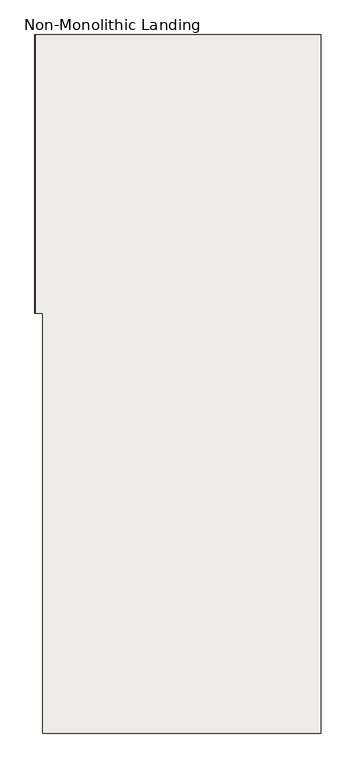
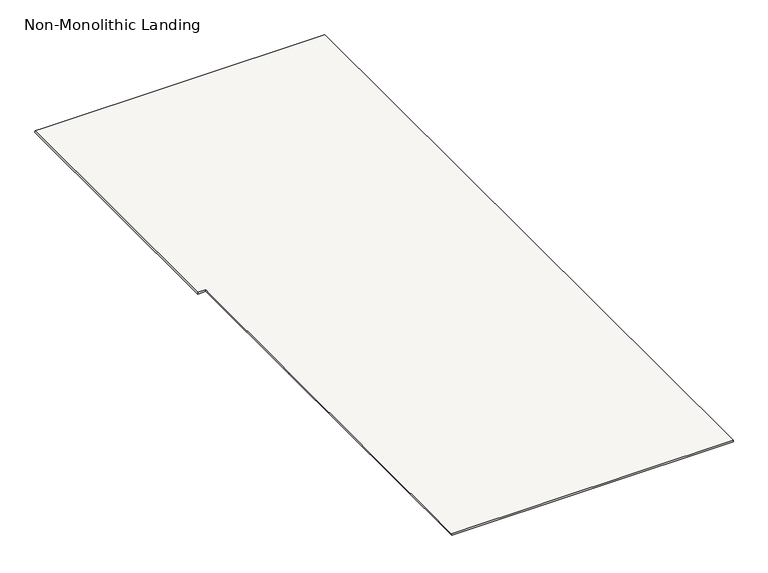
"""IFC4 building model written with IfcOpenShell, lengths in millimetres: slab geometry, Non-Monolithic Landing."""

from ifc_helpers import new_model, si_unit, origin, place, context, project, spatial, faceted_brep, source, transform, mapped, element, save


def non_monolithic_landing_193fae1a(model_context):
    return source(origin(), model_context, "Body", "Brep", [
        faceted_brep([(16318.9400908, 13130.4345331, 9941.1764706), (16318.0900908, 13130.4345331, 9935.1764706), (16318.0900908, 12030.4345331, 9935.1764706), (16318.9400908, 12030.4345331, 9941.1764706), (16350.0, 10370.4345331, 9941.1764706), (17450.0, 10370.4345331, 9941.1764706), (17450.0, 13130.4345331, 9941.1764706), (16350.0, 13130.4345331, 9941.1764706), (16350.0, 12030.4345331, 9941.1764706), (16350.0, 11470.4345331, 9941.1764706), (17450.0, 13130.4345331, 9935.1764706), (17450.0, 10370.4345331, 9935.1764706), (16350.85, 10370.4345331, 9935.1764706), (16350.85, 11470.4345331, 9935.1764706), (16350.0, 11470.4345331, 9935.1764706), (16350.0, 12030.4345331, 9935.1764706), (16350.0, 13130.4345331, 9935.1764706)], [[[0, 1, 2, 3]], [[4, 5, 6, 7, 0, 3, 8, 9]], [[10, 11, 12, 13, 14, 15, 2, 1, 16]], [[9, 8, 15, 14]], [[0, 7, 16, 1]], [[7, 6, 10, 16]], [[6, 5, 11, 10]], [[5, 4, 12, 11]], [[13, 9, 14]], [[9, 13, 12, 4]], [[8, 3, 2, 15]]]),
    ])


if __name__ == "__main__":
    model = new_model("IFC4")
    model_context = context("Model", 3, world=origin())
    ifc_project = project(units=[si_unit("LENGTHUNIT", "METRE", prefix="MILLI")], contexts=[model_context])
    site = spatial("IfcSite", under=ifc_project)
    building = spatial("IfcBuilding", under=site)
    placement = place(None, origin())
    non_monolithic_landing_shape = non_monolithic_landing_193fae1a(model_context)
    element("IfcSlab", 1, ObjectType="Non-Monolithic Landing", at=placement, inside=building, context=model_context, shape_type="MappedRepresentation", body=[
        mapped(non_monolithic_landing_shape, transform((0.0, 0.0, 0.0), x_axis=(1.0, 0.0, 0.0), y_axis=(0.0, 1.0, 0.0), z_axis=(0.0, 0.0, 1.0))),
    ])
    save(model, "model.ifc")

# Revit data of these elements
# Element 1 (IfcSlab, "Non-Monolithic Landing")
#   Materials on its faces: "Steel, Paint Finish, Dark Gray"
# Materials
#   "Steel, Paint Finish, Dark Gray": class "Metal", colour RGB 89 89 89, transparency 0, Description = "Steel, paint finish, dark gray, glossy", Cost = 0
